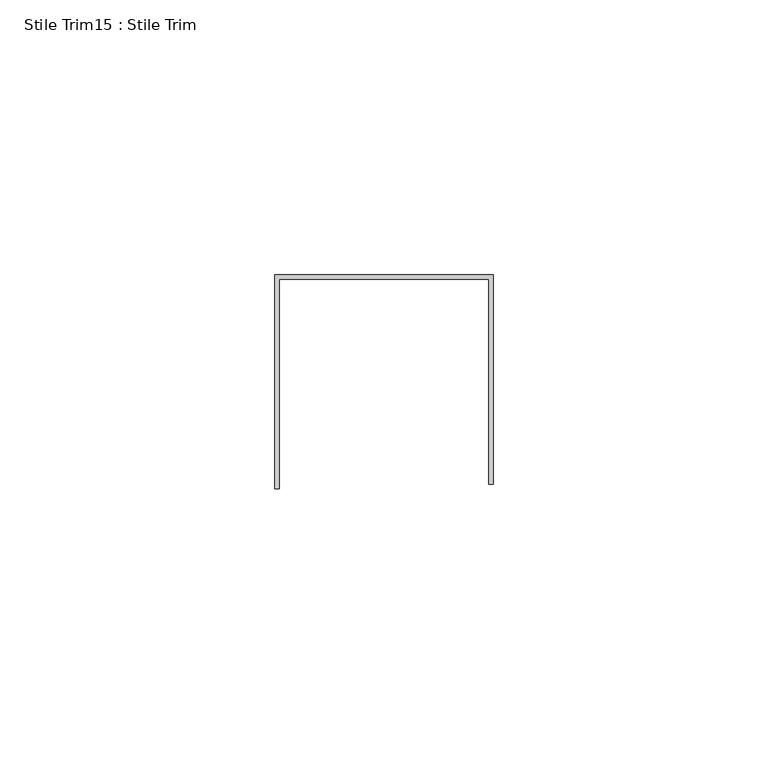
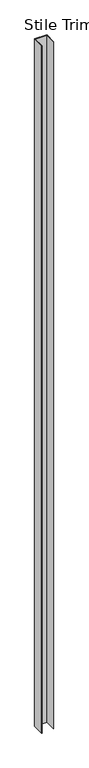
"""IFC4 building model written with IfcOpenShell, lengths in millimetres: proxy geometry, Stile Trim15 : Stile Trim."""

from ifc_helpers import new_model, si_unit, frame, origin, place, context, project, spatial, polyline, outline, extrude, source, transform, mapped, element, save


def stile_trim15_stile_trim_b98e89d7(model_context):
    return source(origin(), model_context, "Body", "SweptSolid", [
        extrude(outline(polyline([(587327.0060739, -532883.0289841), (587366.6808739, -532883.0289841), (587366.6808739, -532921.1289841), (587365.8934739, -532921.1289841), (587365.8934739, -532883.8163841), (587327.7934739, -532883.8163841), (587327.7934739, -532921.9163841), (587327.0060739, -532921.9163841), (587327.0060739, -532883.0289841)])), frame((0.0, 0.0, 50.8), z_axis=(0.0, 0.0, 1.0), x_axis=(1.0, 0.0, 0.0)), (0.0, 0.0, 1.0), 2350.3929688),
    ])


if __name__ == "__main__":
    model = new_model("IFC4")
    model_context = context("Model", 3, world=origin())
    ifc_project = project(units=[si_unit("LENGTHUNIT", "METRE", prefix="MILLI")], contexts=[model_context])
    site = spatial("IfcSite", under=ifc_project)
    building = spatial("IfcBuilding", under=site)
    placement = place(None, origin())
    stile_trim15_stile_trim_shape = stile_trim15_stile_trim_b98e89d7(model_context)
    element("IfcBuildingElementProxy", 1, Name="Stile Trim15 : Stile Trim", ObjectType="Stile Trim15 : Stile Trim", at=placement, inside=building, context=model_context, shape_type="MappedRepresentation", body=[
        mapped(stile_trim15_stile_trim_shape, transform((0.0, 0.0, 0.0), x_axis=(1.0, 0.0, 0.0), y_axis=(0.0, 1.0, 0.0), z_axis=(0.0, 0.0, 1.0))),
    ])
    save(model, "model.ifc")

# Revit data of these elements
# Element 1 (IfcBuildingElementProxy, "Stile Trim15 : Stile Trim")
#   Materials on its faces: "EDGE TRIM BY MTL PANEL MFR."
# Materials
#   "EDGE TRIM BY MTL PANEL MFR.": class "Generic", colour RGB 239 242 240, transparency 0, Cost = 0
